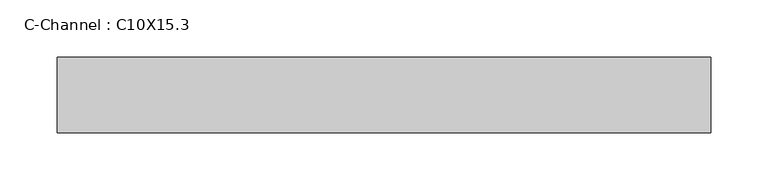
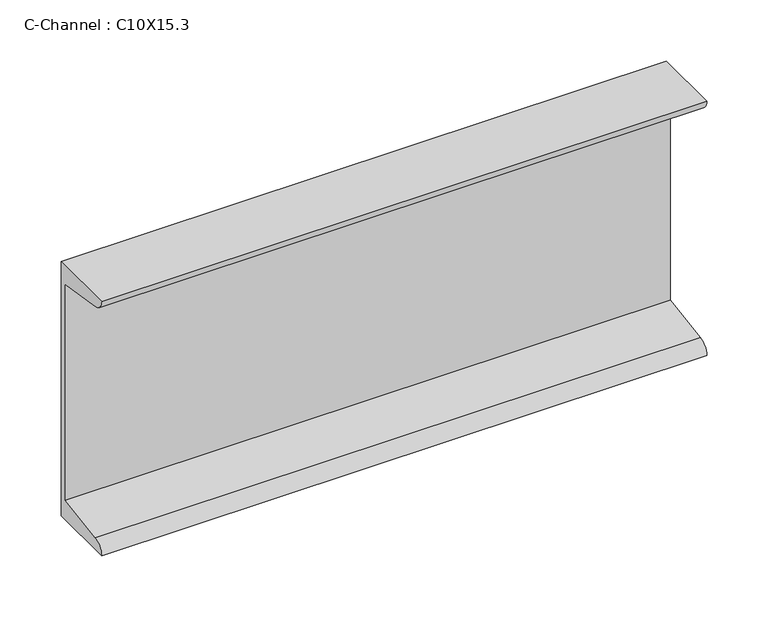
"""IFC4 building model written with IfcOpenShell, lengths in millimetres: beam geometry, C-Channel : C10X15.3."""

from ifc_helpers import new_model, si_unit, point, frame, frame_2d, origin, place, context, project, spatial, polyline, circle_curve, trimmed, segment, composite_curve, outline, extrude, source, transform, mapped, element, save


def c_channel_c10x15_3_bc53fe10(model_context):
    return source(origin(), model_context, "Body", "SweptSolid", [
        extrude(outline(composite_curve([segment(polyline([(16.1036, 127.0), (16.1036, -127.0), (-49.9364, -127.0)]), True, "CONTINUOUS"), segment(trimmed(circle_curve(frame_2d((-38.862, -127.0)), 11.0744), [point((-49.9364, -127.0))], [point((-38.862, -115.9256))], False, "CARTESIAN"), True, "CONTINUOUS"), segment(polyline([(-38.862, -115.9256), (10.0076, -108.1854158), (10.0076, 108.1854158), (-38.862, 115.9256)]), True, "CONTINUOUS"), segment(trimmed(circle_curve(frame_2d((-38.862, 127.0)), 11.0744), [point((-38.862, 115.9256))], [point((-49.9364, 127.0))], False, "CARTESIAN"), True, "CONTINUOUS"), segment(polyline([(-49.9364, 127.0), (16.1036, 127.0)]), True, "CONTINUOUS")], self_intersect=False)), frame((-292.1, 0.0, 0.0), z_axis=(1.0, 0.0, 0.0), x_axis=(0.0, 1.0, 0.0)), (0.0, 0.0, 1.0), 571.4999994),
    ])


if __name__ == "__main__":
    model = new_model("IFC4")
    model_context = context("Model", 3, world=origin())
    ifc_project = project(units=[si_unit("LENGTHUNIT", "METRE", prefix="MILLI")], contexts=[model_context])
    site = spatial("IfcSite", under=ifc_project)
    building = spatial("IfcBuilding", under=site)
    placement = place(None, origin())
    c_channel_c10x15_3_shape = c_channel_c10x15_3_bc53fe10(model_context)
    element("IfcBeam", 1, ObjectType="C-Channel : C10X15.3", at=placement, inside=building, context=model_context, shape_type="MappedRepresentation", body=[
        mapped(c_channel_c10x15_3_shape, transform((0.0, 0.0, 0.0), x_axis=(1.0, 0.0, 0.0), y_axis=(0.0, 1.0, 0.0), z_axis=(0.0, 0.0, 1.0))),
    ])
    save(model, "model.ifc")

# Revit data of these elements
# Type "C-Channel : C10X15.3"
#   Assembly Code = "B10"
#   W = 15.3
#   Length [instance default] = 5' - 0"
#   bf = 0' - 2.6"
#   d = 0' - 10"
#   tf = 0' - 0.436"
#   tw = 0' - 0.24"
#   x = 0' - 0.634"
#   A = 0.0311111 SF
#   Structural Material [instance default] = Steel ASTM A36
# Element 1 (IfcBeam, "C-Channel : C10X15.3")
#   Structural Material = Steel ASTM A992
#   Materials on its faces: "Steel ASTM A992"
# Materials
#   "Steel ASTM A36": class "Metal", colour RGB 199 199 199, transparency 0, Description = "Structural steel, ASTM A36 Grade B, mill finish", Cost = 0
#   "Steel ASTM A992": class "Metal", colour RGB 199 199 199, transparency 0, Description = "Structural steel 50ksi", Cost = 0
